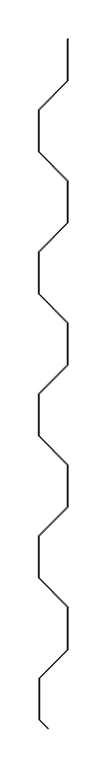
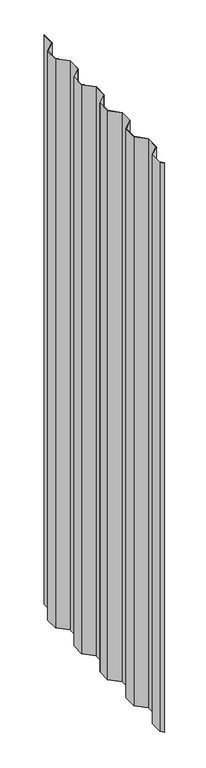
"""IFC4 building model written with IfcOpenShell, lengths in millimetres: proxy geometry, MBCI 7.2-V Panel14 : MBCI 7.2-V Panel-1."""

from ifc_helpers import new_model, si_unit, frame, origin, place, context, project, spatial, polyline, outline, extrude, source, transform, mapped, element, save


def generic_models_2bd7a00a(model_context):
    return source(origin(), model_context, "Body", "SweptSolid", [
        extrude(outline(polyline([(590391.0731614, -531702.4697976), (590391.0731614, -531649.0310327), (590391.6684739, -531648.4357202), (590391.6684739, -531702.7163841), (590354.1780739, -531740.2067841), (590354.1780739, -531793.8253202), (590391.6684739, -531831.3157202), (590391.6684739, -531885.5963841), (590354.1780739, -531923.0867841), (590354.1780739, -531976.7053202), (590391.6684739, -532014.1957202), (590391.6684739, -532068.4763841), (590354.1780739, -532105.9667841), (590354.1780739, -532159.5853202), (590391.6684739, -532197.0757202), (590391.6684739, -532251.3563841), (590354.1780739, -532288.8467841), (590354.1780739, -532342.4653202), (590391.6684739, -532379.9557202), (590391.6684739, -532435.0999841), (590354.7876739, -532471.9807841), (590354.7876739, -532525.0689111), (590365.9181078, -532536.199345), (590365.8630841, -532536.9862203), (590354.1923614, -532525.3154976), (590354.1923614, -532471.7341976), (590391.0731614, -532434.8533976), (590391.0731614, -532380.2023067), (590353.5827614, -532342.7119067), (590353.5827614, -532288.6001976), (590391.0731614, -532251.1097976), (590391.0731614, -532197.3223067), (590353.5827614, -532159.8319067), (590353.5827614, -532105.7201976), (590391.0731614, -532068.2297976), (590391.0731614, -532014.4423067), (590353.5827614, -531976.9519067), (590353.5827614, -531922.8401976), (590391.0731614, -531885.3497976), (590391.0731614, -531831.5623067), (590353.5827614, -531794.0719067), (590353.5827614, -531739.9601976), (590391.0731614, -531702.4697976)])), frame((0.0, 0.0, 6.35), z_axis=(0.0, 0.0, 1.0), x_axis=(1.0, 0.0, 0.0)), (0.0, 0.0, 1.0), 2432.05),
    ])


if __name__ == "__main__":
    model = new_model("IFC4")
    model_context = context("Model", 3, world=origin())
    ifc_project = project(units=[si_unit("LENGTHUNIT", "METRE", prefix="MILLI")], contexts=[model_context])
    site = spatial("IfcSite", under=ifc_project)
    building = spatial("IfcBuilding", under=site)
    placement = place(None, origin())
    generic_models_shape = generic_models_2bd7a00a(model_context)
    element("IfcBuildingElementProxy", 1, Name="MBCI 7.2-V Panel14 : MBCI 7.2-V Panel-1", ObjectType="MBCI 7.2-V Panel14 : MBCI 7.2-V Panel-1", at=placement, inside=building, context=model_context, shape_type="MappedRepresentation", body=[
        mapped(generic_models_shape, transform((0.0, 0.0, 0.0), x_axis=(1.0, 0.0, 0.0), y_axis=(0.0, 1.0, 0.0), z_axis=(0.0, 0.0, 1.0))),
    ])
    save(model, "model.ifc")

# Revit data of these elements
# Element 1 (IfcBuildingElementProxy, "MBCI 7.2-V Panel14 : MBCI 7.2-V Panel-1")
#   Materials on its faces: "MTL PANEL"
# Materials
#   "MTL PANEL": class "Generic", colour RGB 239 242 240, transparency 0, Cost = 0
